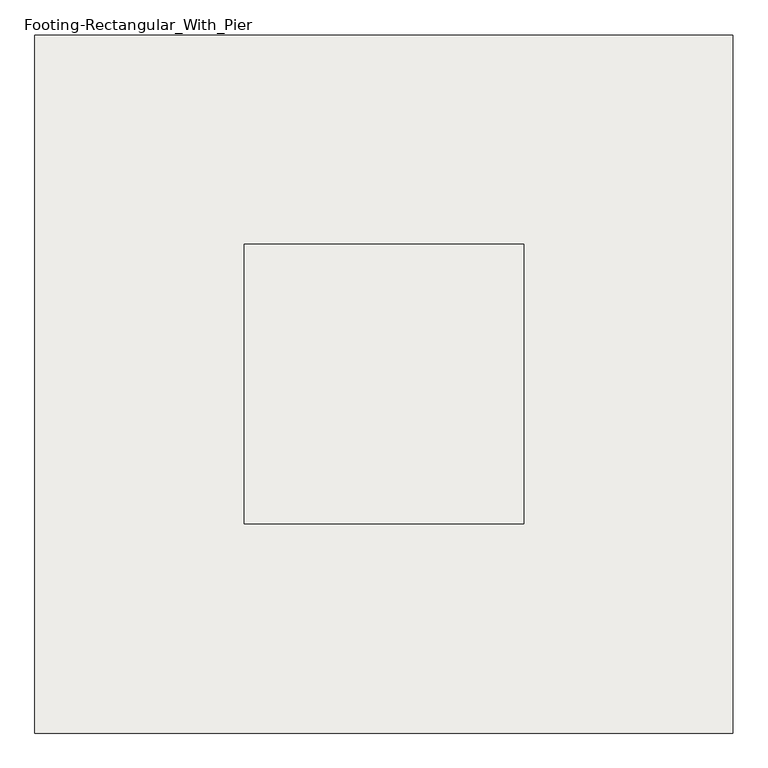
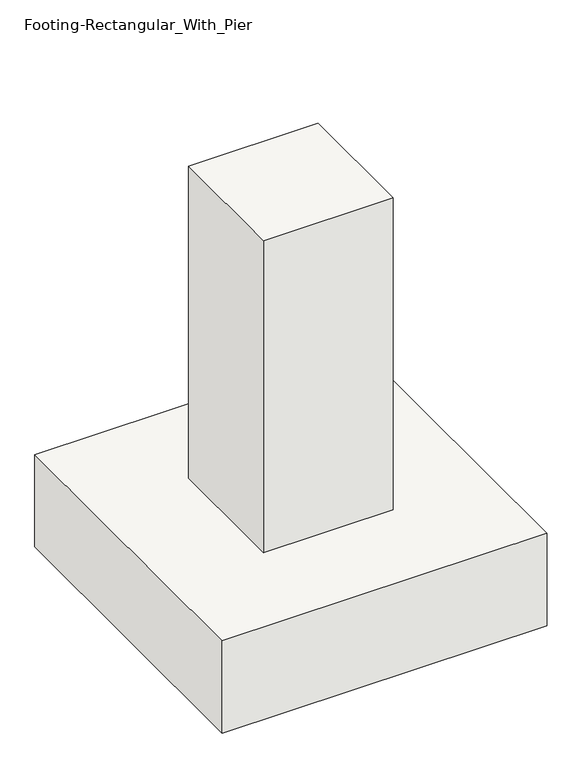
"""IFC4 building model written with IfcOpenShell, lengths in millimetres: slab geometry, Footing-Rectangular_With_Pier."""

from ifc_helpers import new_model, si_unit, frame, origin, origin_with_axes, place, context, project, spatial, polyline, outline, extrude, source, transform, mapped, element, save


def footing_rectangular_with_pier_b4053baf(model_context):
    return source(origin(), model_context, "Body", "SweptSolid", [
        extrude(outline(polyline([(762.0, 762.0), (762.0, -762.0), (-762.0, -762.0), (-762.0, 762.0), (762.0, 762.0)])), frame((0.0, 0.0, -457.2), z_axis=(0.0, 0.0, 1.0), x_axis=(1.0, 0.0, 0.0)), (0.0, 0.0, 1.0), 457.2),
        extrude(outline(polyline([(304.8, 304.8), (304.8, -304.8), (-304.8, -304.8), (-304.8, 304.8), (304.8, 304.8)])), origin_with_axes(), (0.0, 0.0, 1.0), 1549.4),
    ])


if __name__ == "__main__":
    model = new_model("IFC4")
    model_context = context("Model", 3, world=origin())
    ifc_project = project(units=[si_unit("LENGTHUNIT", "METRE", prefix="MILLI")], contexts=[model_context])
    site = spatial("IfcSite", under=ifc_project)
    building = spatial("IfcBuilding", under=site)
    placement = place(None, origin())
    footing_rectangular_with_pier_shape = footing_rectangular_with_pier_b4053baf(model_context)
    element("IfcSlab", 1, ObjectType="Footing-Rectangular_With_Pier : F1 - 5'-0\" x 5'-0\" x 1'-6\"", at=placement, inside=building, context=model_context, shape_type="MappedRepresentation", body=[
        mapped(footing_rectangular_with_pier_shape, transform((0.0, 0.0, 0.0), x_axis=(1.0, 0.0, 0.0), y_axis=(0.0, 1.0, 0.0), z_axis=(0.0, 0.0, 1.0))),
    ])
    save(model, "model.ifc")

# Revit data of these elements
# Type "Footing-Rectangular_With_Pier : F1 - 5'-0\" x 5'-0\" x 1'-6\""
#   Type Mark = "F1"
#   Assembly Code = "A1010100"
#   Width = 1524 mm
#   SteelPlateWidth [instance default] = 406.4 mm
#   SteelPlateThickness [instance default] = 25.4 mm
#   SteelPlateDepth [instance default] = 406.4 mm
#   PierWidth [instance default] = 609.6 mm
#   PierLength [instance default] = 609.6 mm
#   PierDepth [instance default] = 1371.6 mm
#   Length = 1524 mm
#   FootingThickness = 457.2 mm
#   Steel Plate = no
#   Structural Material [instance default] = Concrete - Cast-in-Place Concrete
# Element 1 (IfcSlab, "Footing-Rectangular_With_Pier : F1 - 5'-0\" x 5'-0\" x 1'-6\"")
#   PierDepth = 1549.4 mm
#   Materials on its faces: "Concrete - Cast-in-Place Concrete"
# Materials
#   "Concrete - Cast-in-Place Concrete": class "Concrete", colour RGB 192 192 192, transparency 0
